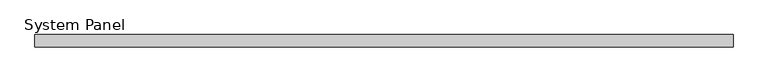
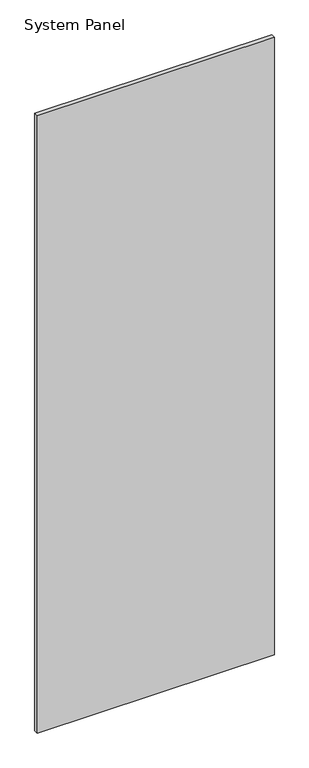
"""IFC4 building model written with IfcOpenShell, lengths in millimetres: plate geometry, System Panel : WWm-Glass-20mm-10mmOffset."""

from ifc_helpers import new_model, si_unit, origin, origin_with_axes, place, context, project, spatial, polyline, outline, extrude, source, transform, mapped, element, save


def system_panel_63faa521(model_context):
    return source(origin(), model_context, "Body", "SweptSolid", [
        extrude(outline(polyline([(572.5751066, 0.0), (-572.5751066, 0.0), (-572.5751066, 20.0), (572.5751066, 20.0), (572.5751066, 0.0)])), origin_with_axes(), (0.0, 0.0, 1.0), 3150.0),
    ])


if __name__ == "__main__":
    model = new_model("IFC4")
    model_context = context("Model", 3, world=origin())
    ifc_project = project(units=[si_unit("LENGTHUNIT", "METRE", prefix="MILLI")], contexts=[model_context])
    site = spatial("IfcSite", under=ifc_project)
    building = spatial("IfcBuilding", under=site)
    placement = place(None, origin())
    system_panel_shape = system_panel_63faa521(model_context)
    element("IfcPlate", 1, ObjectType="System Panel : WWm-Glass-20mm-10mmOffset", at=placement, inside=building, context=model_context, shape_type="MappedRepresentation", body=[
        mapped(system_panel_shape, transform((0.0, 0.0, 0.0), x_axis=(1.0, 0.0, 0.0), y_axis=(0.0, 1.0, 0.0), z_axis=(0.0, 0.0, 1.0))),
    ])
    save(model, "model.ifc")

# Revit data of these elements
# Type "System Panel : WWm-Glass-20mm-10mmOffset"
#   Finish = ""
# Element 1 (IfcPlate, "System Panel : WWm-Glass-20mm-10mmOffset")
#   Materials on its faces: "WW-EC-GL-Storefront"
# Materials
#   "WW-EC-GL-Storefront": class "Glass", colour RGB 236 240 239, transparency 0.85, Description = "Storefront Glass", Cost = 0
